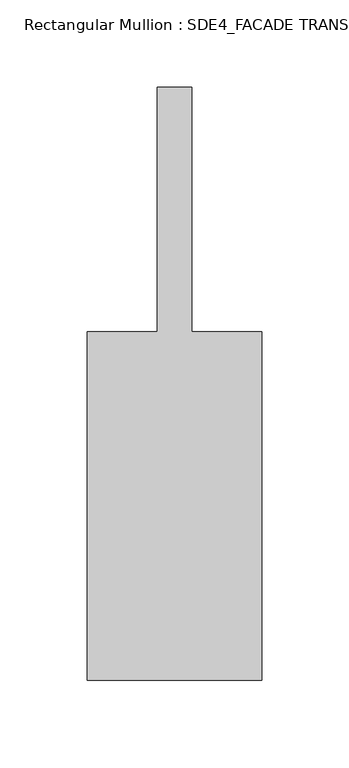
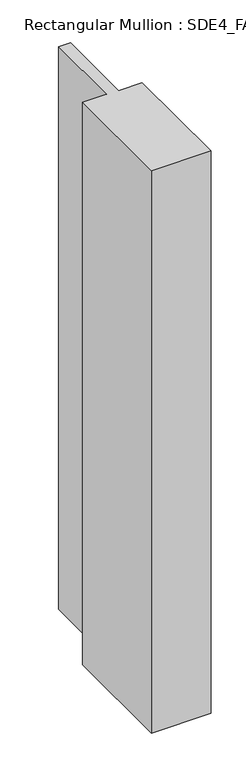
"""IFC4 building model written with IfcOpenShell, lengths in millimetres: member geometry, Rectangular Mullion : SDE4_FACADE TRANSOM TYPE 1."""

from ifc_helpers import new_model, si_unit, frame, origin, place, context, project, spatial, polyline, outline, extrude, source, transform, mapped, element, save


def rectangular_mullion_sde4_facade_transom_type_1_9ddd46d2(model_context):
    return source(origin(), model_context, "Body", "SweptSolid", [
        extrude(outline(polyline([(50.0, -132.5), (-50.0, -132.5), (-50.0, 67.5), (-10.0, 67.5), (-10.0, 207.5), (10.0, 207.5), (10.0, 67.5), (50.0, 67.5), (50.0, -132.5)])), frame((0.0, 0.0, -1000.1632406), z_axis=(0.0, 0.0, 1.0), x_axis=(1.0, 0.0, 0.0)), (0.0, 0.0, 1.0), 1000.1632406),
    ])


if __name__ == "__main__":
    model = new_model("IFC4")
    model_context = context("Model", 3, world=origin())
    ifc_project = project(units=[si_unit("LENGTHUNIT", "METRE", prefix="MILLI")], contexts=[model_context])
    site = spatial("IfcSite", under=ifc_project)
    building = spatial("IfcBuilding", under=site)
    placement = place(None, origin())
    rectangular_mullion_sde4_facade_transom_type_1_shape = rectangular_mullion_sde4_facade_transom_type_1_9ddd46d2(model_context)
    element("IfcMember", 1, ObjectType="Rectangular Mullion : SDE4_FACADE TRANSOM TYPE 1", at=placement, inside=building, context=model_context, shape_type="MappedRepresentation", body=[
        mapped(rectangular_mullion_sde4_facade_transom_type_1_shape, transform((0.0, 0.0, 0.0), x_axis=(1.0, 0.0, 0.0), y_axis=(0.0, 1.0, 0.0), z_axis=(0.0, 0.0, 1.0))),
    ])
    save(model, "model.ifc")

# Revit data of these elements
# Type "Rectangular Mullion : SDE4_FACADE TRANSOM TYPE 1"
#   built-in parameter 1007322 = 1.11549 (stored number, unit not read)
#   built-in parameter 1007321 = 0.164042 (stored number, unit not read)
#   built-in parameter 1007320 = 0.164042 (stored number, unit not read)
